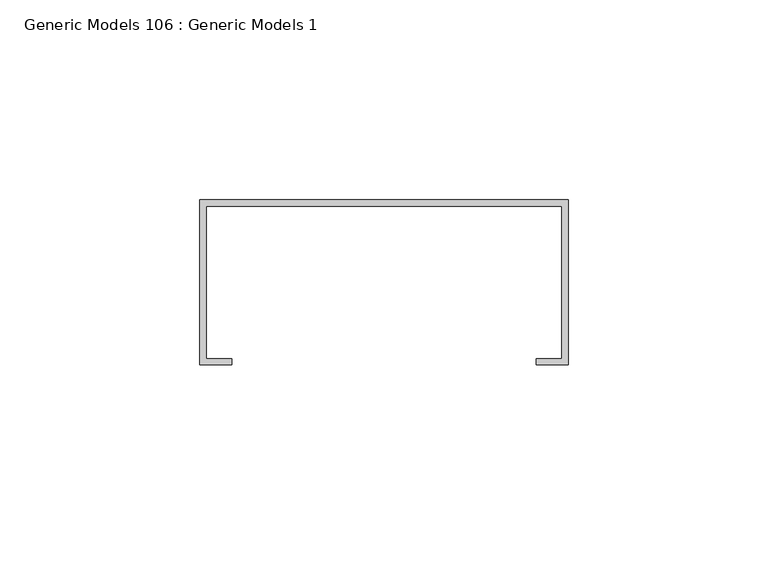
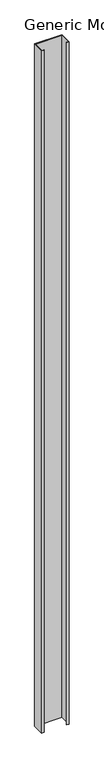
"""IFC4 building model written with IfcOpenShell, lengths in millimetres: proxy geometry, Generic Models 106 : Generic Models 1."""

from ifc_helpers import new_model, si_unit, frame, origin, place, context, project, spatial, polyline, outline, extrude, source, transform, mapped, element, save


def generic_models_106_generic_models_1_274f06fa(model_context):
    return source(origin(), model_context, "Body", "SweptSolid", [
        extrude(outline(polyline([(49691.925, 630.2375), (49784.0, 630.2375), (49784.0, 588.9625), (49776.0625, 588.9625), (49776.0625, 590.55), (49782.4125, 590.55), (49782.4125, 628.65), (49693.5125, 628.65), (49693.5125, 590.55), (49699.8625, 590.55), (49699.8625, 588.9625), (49691.925, 588.9625), (49691.925, 630.2375)])), frame((0.0, 0.0, 1.5875), z_axis=(0.0, 0.0, 1.0), x_axis=(1.0, 0.0, 0.0)), (0.0, 0.0, 1.0), 2428.875),
    ])


if __name__ == "__main__":
    model = new_model("IFC4")
    model_context = context("Model", 3, world=origin())
    ifc_project = project(units=[si_unit("LENGTHUNIT", "METRE", prefix="MILLI")], contexts=[model_context])
    site = spatial("IfcSite", under=ifc_project)
    building = spatial("IfcBuilding", under=site)
    placement = place(None, origin())
    generic_models_106_generic_models_1_shape = generic_models_106_generic_models_1_274f06fa(model_context)
    element("IfcBuildingElementProxy", 1, Name="Generic Models 106 : Generic Models 1", ObjectType="Generic Models 106 : Generic Models 1", at=placement, inside=building, context=model_context, shape_type="MappedRepresentation", body=[
        mapped(generic_models_106_generic_models_1_shape, transform((0.0, 0.0, 0.0), x_axis=(1.0, 0.0, 0.0), y_axis=(0.0, 1.0, 0.0), z_axis=(0.0, 0.0, 1.0))),
    ])
    save(model, "model.ifc")

# Revit data of these elements
# Element 1 (IfcBuildingElementProxy, "Generic Models 106 : Generic Models 1")
#   Materials on its faces: "METAL STUDS (MATCH EXISTING SIZE/GAUGE/SPACING)"
# Materials
#   "METAL STUDS (MATCH EXISTING SIZE/GAUGE/SPACING)": class "Unassigned", colour RGB 210 209 208, transparency 0, Keynote = "M05121300.02", Cost = 0
